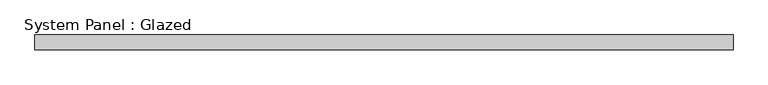
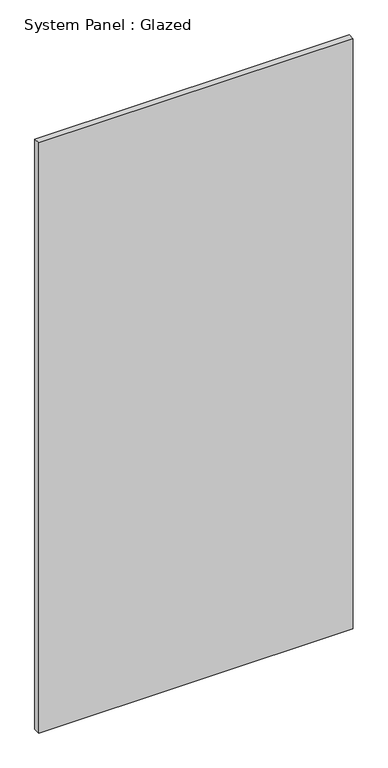
"""IFC4 building model written with IfcOpenShell, lengths in millimetres: plate geometry, System Panel : Glazed."""

import ifcopenshell
import ifcopenshell.guid

model = None  # the IFC model being written
_history = None  # IfcOwnerHistory: only IFC2X3 demands one
_inside = {}  # id of a spatial element -> (the spatial element, [elements in it])
_under = {}  # id of a project, library or spatial element -> (it, [spatial elements below it])
_declared = {}  # id of a project -> (the project, [libraries it declares])
_typed = {}  # id of a type object -> (the type object, [elements of that type])
_made_of = {}  # id of a material, layer set ... -> (it, [elements and type objects made of it])


def new_model(schema):
    """Start an empty IFC model of exactly this schema.

    Asked for "IFC4X3", IfcOpenShell would pick the latest addendum, in which some entities
    have other attributes; the version numbers below select the first issue.
    IFC2X3 requires an IfcOwnerHistory on every rooted entity: one is made here for all.
    """
    global model, _history
    if schema == "IFC4X3":
        model = ifcopenshell.file(schema_version=(4, 3, 0, 0))
    else:
        model = ifcopenshell.file(schema=schema)
    _inside.clear()
    _under.clear()
    _declared.clear()
    _typed.clear()
    _made_of.clear()
    _history = None
    if model.schema == "IFC2X3":
        org = make("IfcOrganization", Name="unknown")
        user = make(
            "IfcPersonAndOrganization",
            ThePerson=make("IfcPerson", FamilyName="unknown"),
            TheOrganization=org,
        )
        app = make(
            "IfcApplication",
            ApplicationDeveloper=org,
            Version="unknown",
            ApplicationFullName="unknown",
            ApplicationIdentifier="unknown",
        )
        _history = make(
            "IfcOwnerHistory",
            OwningUser=user,
            OwningApplication=app,
            ChangeAction="ADDED",
            CreationDate=0,
        )
    return model


def make(cls, **values):
    """One entity of the class cls with the attributes given. An attribute that is None is left unset."""
    return model.create_entity(
        cls, **{name: value for name, value in values.items() if value is not None}
    )


def rooted(cls, **values):
    """An entity with a GlobalId (a new one), such as an element, a storey or a relation."""
    return make(cls, GlobalId=ifcopenshell.guid.new(), OwnerHistory=_history, **values)


def si_unit(unit_type, name, prefix=None):
    """IfcSIUnit, for example si_unit("LENGTHUNIT", "METRE", prefix="MILLI")."""
    return make("IfcSIUnit", UnitType=unit_type, Prefix=prefix, Name=name)


def assignment(units):
    """IfcUnitAssignment: the units of a project."""
    return None if units is None else make("IfcUnitAssignment", Units=units)


def point(xyz):
    """IfcCartesianPoint."""
    return None if xyz is None else make("IfcCartesianPoint", Coordinates=xyz)


def direction(xyz):
    """IfcDirection."""
    return None if xyz is None else make("IfcDirection", DirectionRatios=xyz)


def frame(location, z_axis=None, x_axis=None):
    """IfcAxis2Placement3D, a coordinate frame: its origin and axes. An axis left out is left unset."""
    return make(
        "IfcAxis2Placement3D",
        Location=point(location),
        Axis=direction(z_axis),
        RefDirection=direction(x_axis),
    )


def origin():
    """The frame at (0, 0, 0) with its axes left unset."""
    return frame((0.0, 0.0, 0.0))


def origin_with_axes():
    """The frame at (0, 0, 0) with the z axis (0, 0, 1) and the x axis (1, 0, 0) written out."""
    return frame((0.0, 0.0, 0.0), z_axis=(0.0, 0.0, 1.0), x_axis=(1.0, 0.0, 0.0))


def place(relative_to, where):
    """IfcLocalPlacement: puts the frame where relative to a parent placement (None: the world)."""
    return make(
        "IfcLocalPlacement", PlacementRelTo=relative_to, RelativePlacement=where
    )


def context(
    kind, dimensions, precision=None, world=None, true_north=None, identifier=None
):
    """IfcGeometricRepresentationContext, for example the 3D "Model" context."""
    return make(
        "IfcGeometricRepresentationContext",
        ContextIdentifier=identifier,
        ContextType=kind,
        CoordinateSpaceDimension=dimensions,
        Precision=precision,
        WorldCoordinateSystem=world,
        TrueNorth=true_north,
    )


def project(units=None, contexts=None):
    """IfcProject with its units and contexts."""
    return rooted(
        "IfcProject",
        Name="project",
        RepresentationContexts=contexts,
        UnitsInContext=assignment(units),
    )


def spatial(cls, under=None, at=None, **own):
    """A site, building, storey or space (cls), placed at a placement, below another one or the project."""
    s = rooted(cls, ObjectPlacement=at, **own)
    if under is not None:
        _under.setdefault(under.id(), (under, []))[1].append(s)
    return s


def polyline(points):
    """IfcPolyline through the points."""
    return make("IfcPolyline", Points=[point(p) for p in points])


def outline(outer, holes=None, kind="AREA"):
    """IfcArbitraryClosedProfileDef: a profile drawn as a closed curve; with holes, ...WithVoids."""
    if holes is None:
        return make("IfcArbitraryClosedProfileDef", ProfileType=kind, OuterCurve=outer)
    return make(
        "IfcArbitraryProfileDefWithVoids",
        ProfileType=kind,
        OuterCurve=outer,
        InnerCurves=holes,
    )


def extrude(swept, where, along, depth):
    """IfcExtrudedAreaSolid: the profile swept, set in the frame where, extruded along a direction by depth."""
    return make(
        "IfcExtrudedAreaSolid",
        SweptArea=swept,
        Position=where,
        ExtrudedDirection=direction(along),
        Depth=depth,
    )


def shape(context_of_items, identifier, shape_type, items):
    """IfcShapeRepresentation: the items that make up one representation, for example the "Body"."""
    return make(
        "IfcShapeRepresentation",
        ContextOfItems=context_of_items,
        RepresentationIdentifier=identifier,
        RepresentationType=shape_type,
        Items=items,
    )


def source(mapping_origin, context_of_items, identifier, shape_type, items):
    """IfcRepresentationMap: a shape defined once, which mapped items show again and again."""
    return make(
        "IfcRepresentationMap",
        MappingOrigin=mapping_origin,
        MappedRepresentation=shape(context_of_items, identifier, shape_type, items),
    )


def transform(
    local_origin,
    x_axis=None,
    y_axis=None,
    z_axis=None,
    scale=None,
    scale2=None,
    scale3=None,
    uniform=True,
):
    """IfcCartesianTransformationOperator3D, or its non-uniform kind. x_axis, y_axis, z_axis: its Axis1, 2, 3."""
    if uniform:
        return make(
            "IfcCartesianTransformationOperator3D",
            Axis1=direction(x_axis),
            Axis2=direction(y_axis),
            LocalOrigin=point(local_origin),
            Scale=scale,
            Axis3=direction(z_axis),
        )
    return make(
        "IfcCartesianTransformationOperator3DnonUniform",
        Axis1=direction(x_axis),
        Axis2=direction(y_axis),
        LocalOrigin=point(local_origin),
        Scale=scale,
        Axis3=direction(z_axis),
        Scale2=scale2,
        Scale3=scale3,
    )


def mapped(mapping_source, mapping_target):
    """IfcMappedItem: shows the shape of a source again, moved by a transform."""
    return make(
        "IfcMappedItem", MappingSource=mapping_source, MappingTarget=mapping_target
    )


def made_of(thing, what):
    """Note that an element or type object is made of a material, layer set ...; save() writes the relation."""
    if what is not None:
        _made_of.setdefault(what.id(), (what, []))[1].append(thing)
    return thing


def element(
    cls,
    number,
    at=None,
    inside=None,
    cuts=None,
    type_object=None,
    material=None,
    context=None,
    identifier="Body",
    shape_type=None,
    held_by="IfcProductDefinitionShape",
    body=None,
    shapes=None,
    **own,
):
    """One element of the class cls, such as IfcWall. Its Tag is "e" and its number.

    at: its placement. inside: the storey or other place that contains it. cuts: it is an
    opening in that element (IfcRelVoidsElement). A single representation is given by context,
    identifier, shape_type and body (its items); several are given by shapes. held_by: the class
    of the entity that holds the representations. save() writes the other relations.
    """
    e = rooted(cls, Tag="e%d" % number, ObjectPlacement=at, **own)
    if body is not None:
        shapes = [shape(context, identifier, shape_type, body)]
    if shapes is not None:
        e.Representation = make(held_by, Representations=shapes)
    if inside is not None:
        _inside.setdefault(inside.id(), (inside, []))[1].append(e)
    if cuts is not None:
        rooted(
            "IfcRelVoidsElement", RelatingBuildingElement=cuts, RelatedOpeningElement=e
        )
    if type_object is not None:
        _typed.setdefault(type_object.id(), (type_object, []))[1].append(e)
    return made_of(e, material)


def aggregate(whole, parts):
    """IfcRelAggregates: a whole, such as a stair, and the parts it consists of."""
    return rooted("IfcRelAggregates", RelatingObject=whole, RelatedObjects=parts)


def save(model, path):
    """Write the relations noted so far, then the file.

    IfcRelAggregates (storeys below a building ...), IfcRelContainedInSpatialStructure (elements
    in a storey), IfcRelDefinesByType, IfcRelAssociatesMaterial and IfcRelDeclares: one each for
    every whole, place, type object, material and project.
    """
    for whole, parts in _under.values():
        aggregate(whole, parts)
    for where, things in _inside.values():
        rooted(
            "IfcRelContainedInSpatialStructure",
            RelatedElements=things,
            RelatingStructure=where,
        )
    for kind, things in _typed.values():
        rooted("IfcRelDefinesByType", RelatedObjects=things, RelatingType=kind)
    for what, things in _made_of.values():
        rooted("IfcRelAssociatesMaterial", RelatedObjects=things, RelatingMaterial=what)
    for by, libraries in _declared.values():
        rooted("IfcRelDeclares", RelatingContext=by, RelatedDefinitions=libraries)
    model.write(path)


def system_panel_glazed_aeecb7a7(model_context):
    return source(origin(), model_context, "Body", "SweptSolid", [
        extrude(outline(polyline([(599.0166667, 19.05), (-599.0166667, 19.05), (-599.0166667, 44.45), (599.0166667, 44.45), (599.0166667, 19.05)])), origin_with_axes(), (0.0, 0.0, 1.0), 2374.9),
    ])


if __name__ == "__main__":
    model = new_model("IFC4")
    model_context = context("Model", 3, world=origin())
    ifc_project = project(units=[si_unit("LENGTHUNIT", "METRE", prefix="MILLI")], contexts=[model_context])
    site = spatial("IfcSite", under=ifc_project)
    building = spatial("IfcBuilding", under=site)
    placement = place(None, origin())
    system_panel_glazed_shape = system_panel_glazed_aeecb7a7(model_context)
    element("IfcPlate", 1, ObjectType="System Panel : Glazed", at=placement, inside=building, context=model_context, shape_type="MappedRepresentation", body=[
        mapped(system_panel_glazed_shape, transform((0.0, 0.0, 0.0), x_axis=(1.0, 0.0, 0.0), y_axis=(0.0, 1.0, 0.0), z_axis=(0.0, 0.0, 1.0))),
    ])
    save(model, "model.ifc")

# Revit data of these elements
# Element 1 (IfcPlate, "System Panel : Glazed")
#   Materials on its faces: "Glass"
# Materials
#   "Glass": class "Glass", colour RGB 218 227 224, transparency 0.85, Description = "Soda Lime Glass", Cost = 0
